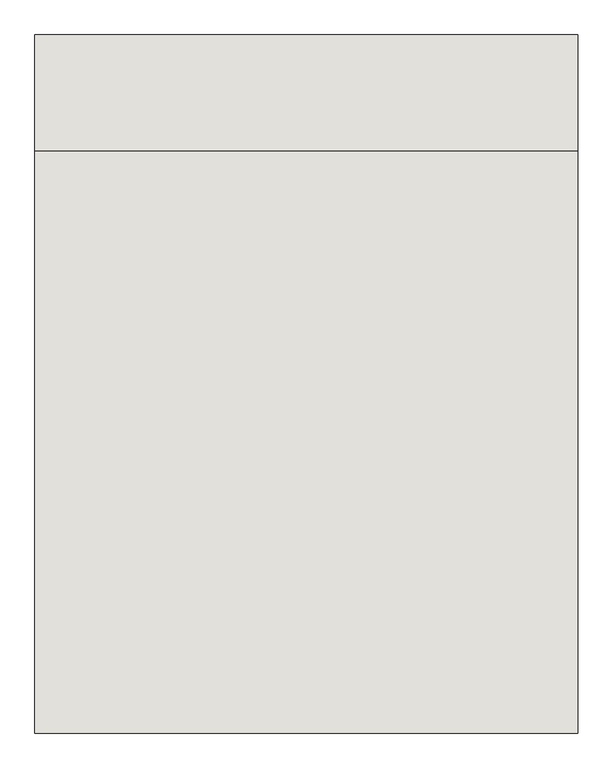
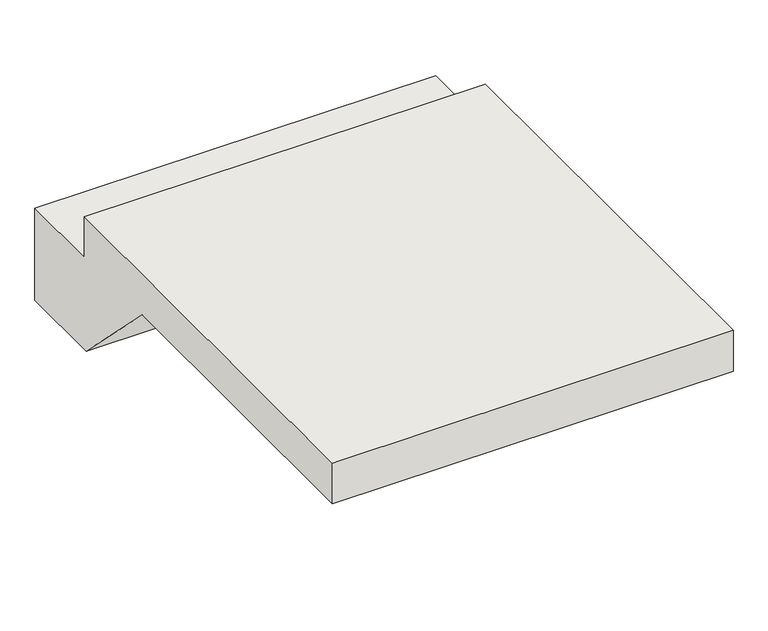
"""IFC4 building model written with IfcOpenShell, lengths in millimetres: wall geometry, 벽 1 : 벽 1."""

from ifc_helpers import new_model, si_unit, frame, origin, place, context, project, spatial, polyline, outline, extrude, source, transform, mapped, element, save


def wall_c40cd3bd(model_context):
    return source(origin(), model_context, "Body", "SweptSolid", [
        extrude(outline(polyline([(40819.5208589, 599.905241), (40819.5208589, 449.905241), (41119.5208589, 449.905241), (41119.5208589, 109.2314637), (40810.1946362, 109.2314637), (40469.5208589, 449.905241), (39319.5208589, 449.905241), (39319.5208589, 599.905241), (40819.5208589, 599.905241)])), frame((21000.0, 0.0, 0.0), z_axis=(1.0, 0.0, 0.0), x_axis=(0.0, 1.0, 0.0)), (0.0, 0.0, 1.0), 1400.0),
    ])


if __name__ == "__main__":
    model = new_model("IFC4")
    model_context = context("Model", 3, world=origin())
    ifc_project = project(units=[si_unit("LENGTHUNIT", "METRE", prefix="MILLI")], contexts=[model_context])
    site = spatial("IfcSite", under=ifc_project)
    building = spatial("IfcBuilding", under=site)
    placement = place(None, origin())
    wall_shape = wall_c40cd3bd(model_context)
    element("IfcWall", 1, ObjectType="벽 1 : 벽 1", at=placement, inside=building, context=model_context, shape_type="MappedRepresentation", body=[
        mapped(wall_shape, transform((0.0, 0.0, 0.0), x_axis=(1.0, 0.0, 0.0), y_axis=(0.0, 1.0, 0.0), z_axis=(0.0, 0.0, 1.0))),
    ])
    save(model, "model.ifc")

# Revit data of these elements
# Element 1 (IfcWall, "벽 1 : 벽 1")
#   Materials on its faces: "A03AC032-00007_Structural Concrete_Type1_25MPa-30Mpa"
# Materials
#   "A03AC032-00007_Structural Concrete_Type1_25MPa-30Mpa": class "Concrete", colour RGB 176 176 176, transparency 0, Keynote = "09910.A1", Description = "Reinf. Conc.", W00) Work Master Code = "A03AC032-00007", W01) Work Master_Lv1 = "Concrete Work", W02) Work Master_Lv2 = "Substructure Work", W03) Work Master_Spec.1 = "Structural Concrete", W04) Work Master_Spec.2 = "Cement Type-1", W05) Work Master_Spec.3 = "25MPa < F'c (Cylinder Strength) ≤ 30MPa", Cost = 0
